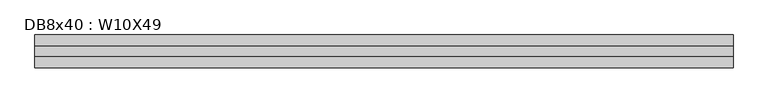
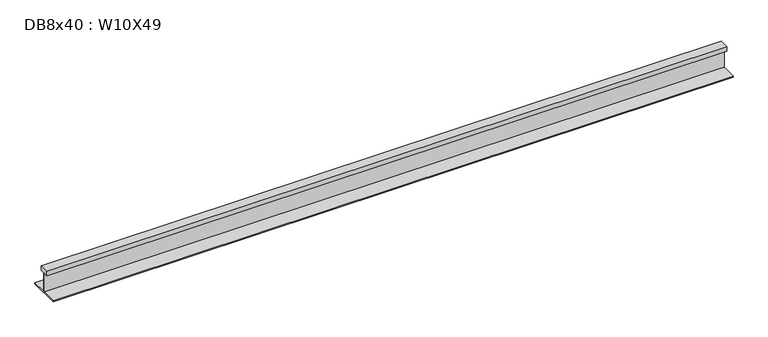
"""IFC4 building model written with IfcOpenShell, lengths in millimetres: beam geometry, DB8x40 : W10X49."""

from ifc_helpers import new_model, si_unit, frame, origin, place, context, project, spatial, polyline, outline, extrude, source, transform, mapped, element, save


def db8x40_w10x49_3fee51fc(model_context):
    return source(origin(), model_context, "Body", "SweptSolid", [
        extrude(outline(polyline([(38.1, 144.3355), (38.1, 106.2355), (2.921, 106.2355), (2.921, -49.53), (127.0, -49.53), (127.0, -59.182), (-127.0, -59.182), (-127.0, -49.53), (-2.921, -49.53), (-2.921, 106.2355), (-38.1, 106.2355), (-38.1, 144.3355), (38.1, 144.3355)])), frame((-2708.529, 0.0, 0.0), z_axis=(1.0, 0.0, 0.0), x_axis=(0.0, 1.0, 0.0)), (0.0, 0.0, 1.0), 5417.058),
    ])


if __name__ == "__main__":
    model = new_model("IFC4")
    model_context = context("Model", 3, world=origin())
    ifc_project = project(units=[si_unit("LENGTHUNIT", "METRE", prefix="MILLI")], contexts=[model_context])
    site = spatial("IfcSite", under=ifc_project)
    building = spatial("IfcBuilding", under=site)
    placement = place(None, origin())
    db8x40_w10x49_shape = db8x40_w10x49_3fee51fc(model_context)
    element("IfcBeam", 1, ObjectType="DB8x40 : W10X49", at=placement, inside=building, context=model_context, shape_type="MappedRepresentation", body=[
        mapped(db8x40_w10x49_shape, transform((0.0, 0.0, 0.0), x_axis=(1.0, 0.0, 0.0), y_axis=(0.0, 1.0, 0.0), z_axis=(0.0, 0.0, 1.0))),
    ])
    save(model, "model.ifc")

# Revit data of these elements
# Type "DB8x40 : W10X49"
#   Assembly Code = "B10"
#   W = 53
#   Length [instance default] = 5' - 0"
#   bf = 0' - 10"
#   d = 1' - 0.1"
#   k = 0' - 1 3/8"
#   k2 = 0' - 0.8"
#   tf = 0' - 0.575"
#   tw = 0' - 0.345"
#   A = 0.108333 SF
#   Structural Material [instance default] = Steel ASTM A992
# Element 1 (IfcBeam, "DB8x40 : W10X49")
#   Materials on its faces: "Steel ASTM A992"
# Materials
#   "Steel ASTM A992": class "Metal", colour RGB 199 199 199, transparency 0, Description = "Structural steel 50ksi", Cost = 0
